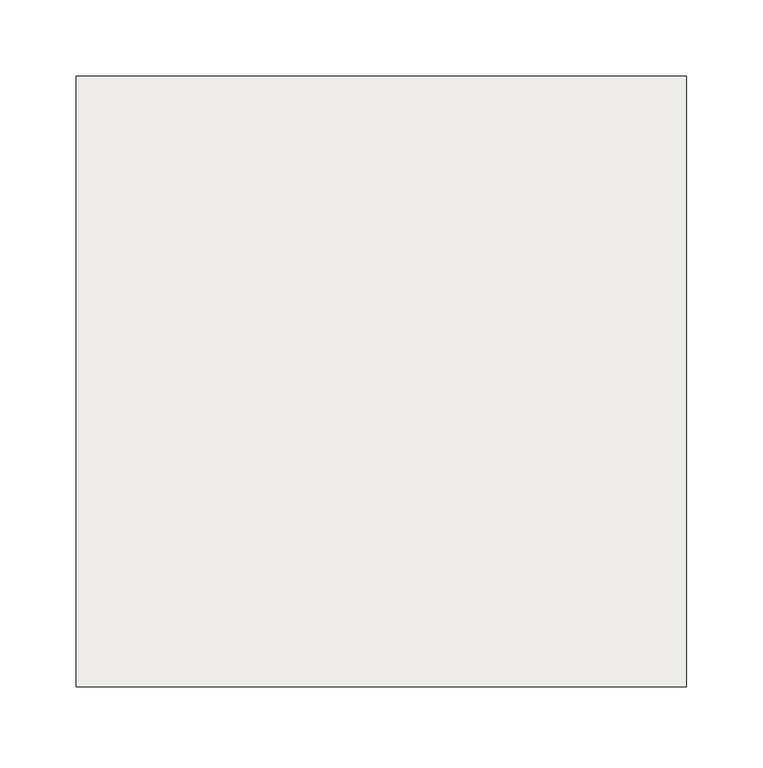
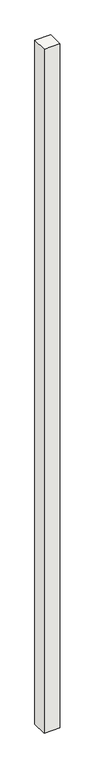
"""IFC4 building model written with IfcOpenShell, lengths in millimetres: footing geometry, NLRS_17_SFO_TLB_funderingspaal geheid beton prefab-AV-MMBPC_gen_rsf : heipaal beton prefab_gen__bxh 400x400."""

from ifc_helpers import new_model, si_unit, frame, origin, place, context, project, spatial, polyline, outline, extrude, source, transform, mapped, element, save


def footing_c32f4c5b(model_context):
    return source(origin(), model_context, "Body", "SweptSolid", [
        extrude(outline(polyline([(200.0, -200.0), (-200.0, -200.0), (-200.0, 200.0), (200.0, 200.0), (200.0, -200.0)])), frame((0.0, 0.0, -20000.0), z_axis=(0.0, 0.0, 1.0), x_axis=(1.0, 0.0, 0.0)), (0.0, 0.0, 1.0), 18290.0),
    ])


if __name__ == "__main__":
    model = new_model("IFC4")
    model_context = context("Model", 3, world=origin())
    ifc_project = project(units=[si_unit("LENGTHUNIT", "METRE", prefix="MILLI")], contexts=[model_context])
    site = spatial("IfcSite", under=ifc_project)
    building = spatial("IfcBuilding", under=site)
    placement = place(None, origin())
    footing_shape = footing_c32f4c5b(model_context)
    element("IfcFooting", 1, ObjectType="NLRS_17_SFO_TLB_funderingspaal geheid beton prefab-AV-MMBPC_gen_rsf : heipaal beton prefab_gen__bxh 400x400", at=placement, inside=building, context=model_context, shape_type="MappedRepresentation", body=[
        mapped(footing_shape, transform((0.0, 0.0, 0.0), x_axis=(1.0, 0.0, 0.0), y_axis=(0.0, 1.0, 0.0), z_axis=(0.0, 0.0, 1.0))),
    ])
    save(model, "model.ifc")

# Revit data of these elements
# Type "NLRS_17_SFO_TLB_funderingspaal geheid beton prefab-AV-MMBPC_gen_rsf : heipaal beton prefab_gen__bxh 400x400"
#   IfcExportAs = "IfcPile"
#   Type Comments = "prefab heipaal 400x400"
#   Model = " "
#   Manufacturer = " "
#   Description = "prefab heipaal 400x400"
#   Assembly Code = "17.21"
#   Width = 400 mm
#   Slanted Angle [instance default] = 0.00°
#   NLRS_S_draagvermogen_trek [instance default] = 0.00 kN
#   NLRS_S_draagvermogen_druk [instance default] = 0.00 kN
#   NLRS_C_lengte [instance default] = 1660 mm
#   NLRS_C_hoogte = 400 mm
#   NLRS_C_breedte = 400 mm
#   Height [instance default] = 1660 mm
#   Length [instance default] = 1660 mm
#   Angle [instance default] = 0.00°
#   Slanted [instance default] = 0
#   Structural Material = NLRS_f2_beton prefab_gen_rsf
#   Keynote = ""
# Element 1 (IfcFooting, "NLRS_17_SFO_TLB_funderingspaal geheid beton prefab-AV-MMBPC_gen_rsf : heipaal beton prefab_gen__bxh 400x400")
#   NLRS_C_lengte = 18290 mm
#   Height = 18290 mm
#   Length = 18290 mm
#   Materials on its faces: "NLRS_f2_beton prefab_gen_rsf"
# Materials
#   "NLRS_f2_beton prefab_gen_rsf": class "F - Niet gebakken kunststeen", colour RGB 129 133 118, transparency 0, Keynote = "f2", Manufacturer = "Revit Standards Foundation", URL = "www.revitstandards.org", Description = "beton prefab", Cost = 0
